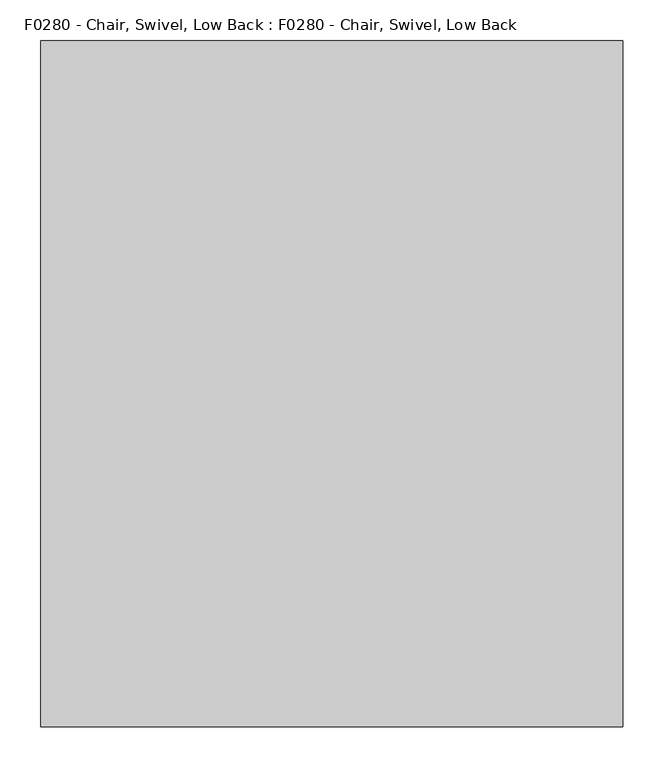
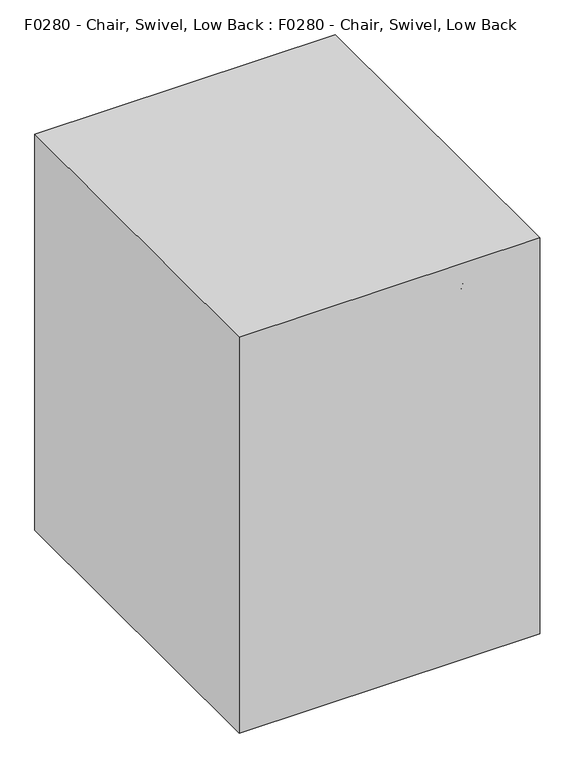
"""IFC4 building model written with IfcOpenShell, lengths in millimetres: proxy geometry, F0280 - Chair, Swivel, Low Back : F0280 - Chair, Swivel, Low Back."""

import ifcopenshell
import ifcopenshell.guid

model = None  # the IFC model being written
_history = None  # IfcOwnerHistory: only IFC2X3 demands one
_inside = {}  # id of a spatial element -> (the spatial element, [elements in it])
_under = {}  # id of a project, library or spatial element -> (it, [spatial elements below it])
_declared = {}  # id of a project -> (the project, [libraries it declares])
_typed = {}  # id of a type object -> (the type object, [elements of that type])
_made_of = {}  # id of a material, layer set ... -> (it, [elements and type objects made of it])


def new_model(schema):
    """Start an empty IFC model of exactly this schema.

    Asked for "IFC4X3", IfcOpenShell would pick the latest addendum, in which some entities
    have other attributes; the version numbers below select the first issue.
    IFC2X3 requires an IfcOwnerHistory on every rooted entity: one is made here for all.
    """
    global model, _history
    if schema == "IFC4X3":
        model = ifcopenshell.file(schema_version=(4, 3, 0, 0))
    else:
        model = ifcopenshell.file(schema=schema)
    _inside.clear()
    _under.clear()
    _declared.clear()
    _typed.clear()
    _made_of.clear()
    _history = None
    if model.schema == "IFC2X3":
        org = make("IfcOrganization", Name="unknown")
        user = make(
            "IfcPersonAndOrganization",
            ThePerson=make("IfcPerson", FamilyName="unknown"),
            TheOrganization=org,
        )
        app = make(
            "IfcApplication",
            ApplicationDeveloper=org,
            Version="unknown",
            ApplicationFullName="unknown",
            ApplicationIdentifier="unknown",
        )
        _history = make(
            "IfcOwnerHistory",
            OwningUser=user,
            OwningApplication=app,
            ChangeAction="ADDED",
            CreationDate=0,
        )
    return model


def make(cls, **values):
    """One entity of the class cls with the attributes given. An attribute that is None is left unset."""
    return model.create_entity(
        cls, **{name: value for name, value in values.items() if value is not None}
    )


def rooted(cls, **values):
    """An entity with a GlobalId (a new one), such as an element, a storey or a relation."""
    return make(cls, GlobalId=ifcopenshell.guid.new(), OwnerHistory=_history, **values)


def si_unit(unit_type, name, prefix=None):
    """IfcSIUnit, for example si_unit("LENGTHUNIT", "METRE", prefix="MILLI")."""
    return make("IfcSIUnit", UnitType=unit_type, Prefix=prefix, Name=name)


def assignment(units):
    """IfcUnitAssignment: the units of a project."""
    return None if units is None else make("IfcUnitAssignment", Units=units)


def point(xyz):
    """IfcCartesianPoint."""
    return None if xyz is None else make("IfcCartesianPoint", Coordinates=xyz)


def direction(xyz):
    """IfcDirection."""
    return None if xyz is None else make("IfcDirection", DirectionRatios=xyz)


def frame(location, z_axis=None, x_axis=None):
    """IfcAxis2Placement3D, a coordinate frame: its origin and axes. An axis left out is left unset."""
    return make(
        "IfcAxis2Placement3D",
        Location=point(location),
        Axis=direction(z_axis),
        RefDirection=direction(x_axis),
    )


def frame_2d(location, x_axis=None):
    """IfcAxis2Placement2D, a coordinate frame in the plane: its origin and x axis."""
    return make(
        "IfcAxis2Placement2D", Location=point(location), RefDirection=direction(x_axis)
    )


def origin():
    """The frame at (0, 0, 0) with its axes left unset."""
    return frame((0.0, 0.0, 0.0))


def origin_with_axes():
    """The frame at (0, 0, 0) with the z axis (0, 0, 1) and the x axis (1, 0, 0) written out."""
    return frame((0.0, 0.0, 0.0), z_axis=(0.0, 0.0, 1.0), x_axis=(1.0, 0.0, 0.0))


def origin_2d():
    """The frame at (0, 0) in the plane with its x axis left unset."""
    return frame_2d((0.0, 0.0))


def place(relative_to, where):
    """IfcLocalPlacement: puts the frame where relative to a parent placement (None: the world)."""
    return make(
        "IfcLocalPlacement", PlacementRelTo=relative_to, RelativePlacement=where
    )


def context(
    kind, dimensions, precision=None, world=None, true_north=None, identifier=None
):
    """IfcGeometricRepresentationContext, for example the 3D "Model" context."""
    return make(
        "IfcGeometricRepresentationContext",
        ContextIdentifier=identifier,
        ContextType=kind,
        CoordinateSpaceDimension=dimensions,
        Precision=precision,
        WorldCoordinateSystem=world,
        TrueNorth=true_north,
    )


def project(units=None, contexts=None):
    """IfcProject with its units and contexts."""
    return rooted(
        "IfcProject",
        Name="project",
        RepresentationContexts=contexts,
        UnitsInContext=assignment(units),
    )


def spatial(cls, under=None, at=None, **own):
    """A site, building, storey or space (cls), placed at a placement, below another one or the project."""
    s = rooted(cls, ObjectPlacement=at, **own)
    if under is not None:
        _under.setdefault(under.id(), (under, []))[1].append(s)
    return s


def polyline(points):
    """IfcPolyline through the points."""
    return make("IfcPolyline", Points=[point(p) for p in points])


def circle_curve(where, radius):
    """IfcCircle in the frame where."""
    return make("IfcCircle", Position=where, Radius=radius)


def ellipse_curve(where, semi_axis1, semi_axis2):
    """IfcEllipse in the frame where."""
    return make(
        "IfcEllipse", Position=where, SemiAxis1=semi_axis1, SemiAxis2=semi_axis2
    )


def trimmed(basis, trim1, trim2, sense, master):
    """IfcTrimmedCurve: the piece of a basis curve between two trims."""
    return make(
        "IfcTrimmedCurve",
        BasisCurve=basis,
        Trim1=trim1,
        Trim2=trim2,
        SenseAgreement=sense,
        MasterRepresentation=master,
    )


def segment(curve, same_sense, transition):
    """IfcCompositeCurveSegment."""
    return make(
        "IfcCompositeCurveSegment",
        Transition=transition,
        SameSense=same_sense,
        ParentCurve=curve,
    )


def composite_curve(segments, self_intersect=None):
    """IfcCompositeCurve: segments joined end to end."""
    return make("IfcCompositeCurve", Segments=segments, SelfIntersect=self_intersect)


def outline(outer, holes=None, kind="AREA"):
    """IfcArbitraryClosedProfileDef: a profile drawn as a closed curve; with holes, ...WithVoids."""
    if holes is None:
        return make("IfcArbitraryClosedProfileDef", ProfileType=kind, OuterCurve=outer)
    return make(
        "IfcArbitraryProfileDefWithVoids",
        ProfileType=kind,
        OuterCurve=outer,
        InnerCurves=holes,
    )


def extrude(swept, where, along, depth):
    """IfcExtrudedAreaSolid: the profile swept, set in the frame where, extruded along a direction by depth."""
    return make(
        "IfcExtrudedAreaSolid",
        SweptArea=swept,
        Position=where,
        ExtrudedDirection=direction(along),
        Depth=depth,
    )


def shape(context_of_items, identifier, shape_type, items):
    """IfcShapeRepresentation: the items that make up one representation, for example the "Body"."""
    return make(
        "IfcShapeRepresentation",
        ContextOfItems=context_of_items,
        RepresentationIdentifier=identifier,
        RepresentationType=shape_type,
        Items=items,
    )


def source(mapping_origin, context_of_items, identifier, shape_type, items):
    """IfcRepresentationMap: a shape defined once, which mapped items show again and again."""
    return make(
        "IfcRepresentationMap",
        MappingOrigin=mapping_origin,
        MappedRepresentation=shape(context_of_items, identifier, shape_type, items),
    )


def transform(
    local_origin,
    x_axis=None,
    y_axis=None,
    z_axis=None,
    scale=None,
    scale2=None,
    scale3=None,
    uniform=True,
):
    """IfcCartesianTransformationOperator3D, or its non-uniform kind. x_axis, y_axis, z_axis: its Axis1, 2, 3."""
    if uniform:
        return make(
            "IfcCartesianTransformationOperator3D",
            Axis1=direction(x_axis),
            Axis2=direction(y_axis),
            LocalOrigin=point(local_origin),
            Scale=scale,
            Axis3=direction(z_axis),
        )
    return make(
        "IfcCartesianTransformationOperator3DnonUniform",
        Axis1=direction(x_axis),
        Axis2=direction(y_axis),
        LocalOrigin=point(local_origin),
        Scale=scale,
        Axis3=direction(z_axis),
        Scale2=scale2,
        Scale3=scale3,
    )


def mapped(mapping_source, mapping_target):
    """IfcMappedItem: shows the shape of a source again, moved by a transform."""
    return make(
        "IfcMappedItem", MappingSource=mapping_source, MappingTarget=mapping_target
    )


def made_of(thing, what):
    """Note that an element or type object is made of a material, layer set ...; save() writes the relation."""
    if what is not None:
        _made_of.setdefault(what.id(), (what, []))[1].append(thing)
    return thing


def element(
    cls,
    number,
    at=None,
    inside=None,
    cuts=None,
    type_object=None,
    material=None,
    context=None,
    identifier="Body",
    shape_type=None,
    held_by="IfcProductDefinitionShape",
    body=None,
    shapes=None,
    **own,
):
    """One element of the class cls, such as IfcWall. Its Tag is "e" and its number.

    at: its placement. inside: the storey or other place that contains it. cuts: it is an
    opening in that element (IfcRelVoidsElement). A single representation is given by context,
    identifier, shape_type and body (its items); several are given by shapes. held_by: the class
    of the entity that holds the representations. save() writes the other relations.
    """
    e = rooted(cls, Tag="e%d" % number, ObjectPlacement=at, **own)
    if body is not None:
        shapes = [shape(context, identifier, shape_type, body)]
    if shapes is not None:
        e.Representation = make(held_by, Representations=shapes)
    if inside is not None:
        _inside.setdefault(inside.id(), (inside, []))[1].append(e)
    if cuts is not None:
        rooted(
            "IfcRelVoidsElement", RelatingBuildingElement=cuts, RelatedOpeningElement=e
        )
    if type_object is not None:
        _typed.setdefault(type_object.id(), (type_object, []))[1].append(e)
    return made_of(e, material)


def aggregate(whole, parts):
    """IfcRelAggregates: a whole, such as a stair, and the parts it consists of."""
    return rooted("IfcRelAggregates", RelatingObject=whole, RelatedObjects=parts)


def save(model, path):
    """Write the relations noted so far, then the file.

    IfcRelAggregates (storeys below a building ...), IfcRelContainedInSpatialStructure (elements
    in a storey), IfcRelDefinesByType, IfcRelAssociatesMaterial and IfcRelDeclares: one each for
    every whole, place, type object, material and project.
    """
    for whole, parts in _under.values():
        aggregate(whole, parts)
    for where, things in _inside.values():
        rooted(
            "IfcRelContainedInSpatialStructure",
            RelatedElements=things,
            RelatingStructure=where,
        )
    for kind, things in _typed.values():
        rooted("IfcRelDefinesByType", RelatedObjects=things, RelatingType=kind)
    for what, things in _made_of.values():
        rooted("IfcRelAssociatesMaterial", RelatedObjects=things, RelatingMaterial=what)
    for by, libraries in _declared.values():
        rooted("IfcRelDeclares", RelatingContext=by, RelatedDefinitions=libraries)
    model.write(path)


def plane_surface(at):
    """IfcPlane: the flat surface through the origin of the frame at, square to its z axis."""
    return make("IfcPlane", Position=at)


def cylinder_surface(at, radius):
    """IfcCylindricalSurface: all points at the distance radius from the z axis of the frame at."""
    return make("IfcCylindricalSurface", Position=at, Radius=radius)


def revolved_surface(curve, axis_point, axis_direction):
    """IfcSurfaceOfRevolution: the curve turned about the line through axis_point along axis_direction."""
    return make(
        "IfcSurfaceOfRevolution",
        SweptCurve=make("IfcArbitraryOpenProfileDef", ProfileType="CURVE", Curve=curve),
        AxisPosition=make("IfcAxis1Placement", Location=point(axis_point), Axis=direction(axis_direction)),
    )


def advanced_brep(points, edges, surfaces, faces):
    """IfcAdvancedBrep: a solid bounded by faces that lie on surfaces and meet in shared edges.

    An edge is (start, end): straight between two places in points (the first is 0);
    or (start, end, curve); or (start, end, curve, False) where it runs against its curve.
    A face is (place in surfaces, loops), or (place, loops, False) where it looks against
    its surface's normal. A loop lists edges by number (the first is 1), with a minus sign
    where the edge is run from its end to its start. The first loop is the outer one.
    """
    corners = [point(p) for p in points]
    vertices = [make("IfcVertexPoint", VertexGeometry=c) for c in corners]
    made = []
    for start, end, *more in edges:
        made.append(
            make(
                "IfcEdgeCurve",
                EdgeStart=vertices[start],
                EdgeEnd=vertices[end],
                EdgeGeometry=more[0] if more else make("IfcPolyline", Points=[corners[start], corners[end]]),
                SameSense=more[1] if len(more) > 1 else True,
            )
        )
    hull = []
    for where, loops, *sense in faces:
        bounds = []
        for j, loop in enumerate(loops):
            ring = [make("IfcOrientedEdge", EdgeElement=made[abs(k) - 1], Orientation=k > 0) for k in loop]
            bounds.append(
                make(
                    "IfcFaceOuterBound" if j == 0 else "IfcFaceBound",
                    Bound=make("IfcEdgeLoop", EdgeList=ring),
                    Orientation=True,
                )
            )
        hull.append(make("IfcAdvancedFace", Bounds=bounds, FaceSurface=surfaces[where], SameSense=sense[0] if sense else True))
    return make("IfcAdvancedBrep", Outer=make("IfcClosedShell", CfsFaces=hull))


def f0280_chair_swivel_low_back_f0280_chair_swivel_low_back_8651f157(model_context):
    return source(origin(), model_context, "Body", "SolidModel", [
        advanced_brep(
        [(20.5891067, 0.9088165, 158.3164474), (12.606954, -16.2089653, 158.3164474), (12.606954, -16.2089653, 212.7487443), (20.5891067, 0.9088165, 212.7487443), (283.7284885, -121.7950923, 86.0096871), (283.7284885, -121.7950923, 57.6571213), (275.3053581, -138.7072429, 86.2220806), (287.501904, -133.9556376, 82.2734822), (275.3053581, -138.7072429, 57.8258095), (287.501904, -133.9556376, 54.689734)],
        [
            (0, 1),
            (1, 2),
            (2, 3),
            (3, 0),
            (3, 4),
            (4, 5),
            (5, 0),
            (2, 6),
            (6, 7, ellipse_curve(frame((278.918781, -129.9532617, 86.4074773), z_axis=(0.3625792018206629, -0.16907345849670724, 0.9164881276039822), x_axis=(0.8306203267741233, -0.3873246193939933, -0.40006188516396646)), 10.333389, 9.4704283)),
            (7, 4, ellipse_curve(frame((278.918781, -129.9532617, 86.4074773), z_axis=(0.3625792018206629, -0.16907345849670724, 0.9164881276039822), x_axis=(0.8306203267741233, -0.3873246193939933, -0.40006188516396646)), 10.333389, 9.4704283)),
            (1, 8),
            (8, 6),
            (5, 9, ellipse_curve(frame((278.918781, -129.9532617, 57.9730562), z_axis=(-0.2968743688836678, 0.13843479172039067, -0.9448287768380342), x_axis=(0.8563056778646188, -0.3993018953098915, -0.3275646233321667)), 10.0234334, 9.4704283)),
            (9, 8, ellipse_curve(frame((278.918781, -129.9532617, 57.9730562), z_axis=(-0.2968743688836678, 0.13843479172039067, -0.9448287768380342), x_axis=(0.8563056778646188, -0.3993018953098915, -0.3275646233321667)), 10.0234334, 9.4704283)),
            (9, 7),
        ],
        [
            plane_surface(frame((16.5980304, -7.6500744, 185.5325958), z_axis=(-0.9063077870366449, 0.42261826174071043, 0.0), x_axis=(-0.42261826174071043, -0.9063077870366449, 0.0))),
            plane_surface(frame((20.5891067, 0.9088165, 185.5325958), z_axis=(0.4226182617407104, 0.9063077870366448, 0.0), x_axis=(0.0, 0.0, 1.0))),
            plane_surface(frame((16.5980304, -7.6500744, 212.7487443), z_axis=(0.36257920182066294, -0.16907345849670727, 0.9164881276039825), x_axis=(-0.42261826174071043, -0.9063077870366449, 0.0))),
            plane_surface(frame((12.606954, -16.2089653, 185.5325958), z_axis=(-0.4226182617407102, -0.906307787036645, 0.0), x_axis=(0.0, 0.0, -1.0))),
            plane_surface(frame((16.5980304, -7.6500744, 158.3164474), z_axis=(-0.29687436888366786, 0.1384347917203907, -0.9448287768380345), x_axis=(0.42261826174071043, 0.9063077870366449, 0.0))),
            cylinder_surface(frame((278.918781, -129.9532617, 0.0), z_axis=(0.0, 0.0, -1.0000000000000002), x_axis=(-0.9063077870366449, 0.42261826174071043, 0.0)), 9.4704283),
        ],
        [
            (0, [[1, 2, 3, 4]]),
            (1, [[-4, 5, 6, 7]]),
            (2, [[-3, 8, 9, 10, -5]]),
            (3, [[-2, 11, 12, -8]]),
            (4, [[-1, -7, 13, 14, -11]]),
            (5, [[15, -9, -12, -14]]),
            (5, [[-15, -13, -6, -10]]),
        ],
    ),
        extrude(outline(composite_curve([segment(trimmed(circle_curve(frame_2d((-0.4565328, 0.2009494)), 25.4), [point((24.9434672, 0.2009494))], [point((-25.8565328, 0.2009494))], False, "CARTESIAN"), True, "CONTINUOUS"), segment(trimmed(circle_curve(frame_2d((-0.4565328, 0.2009494)), 25.4), [point((-25.8565328, 0.2009494))], [point((24.9434672, 0.2009494))], False, "CARTESIAN"), True, "CONTINUOUS")], self_intersect=False)), frame((0.0, 0.0, 154.0271692), z_axis=(0.0, 0.0, 1.0), x_axis=(1.0, 0.0, 0.0)), (0.0, 0.0, 1.0), 58.7215752),
        advanced_brep(
        [(-229.5082147, -191.2947504, 328.6387079), (232.0214447, -190.8605661, 328.5937403), (236.3508412, -215.7557493, 331.1720849), (-229.5082147, -216.926585, 331.293346), (-229.5082147, -284.2177228, 855.6310718), (-229.5082147, -307.3958289, 844.3699241), (236.3508412, -306.337077, 844.8843217), (232.0214447, -283.8251028, 855.8218273)],
        [
            (0, 1, circle_curve(frame((0.0, 1130.5045098, 191.7425871), z_axis=(0.0, 0.10301698777210262, 0.9946795967699159), x_axis=(-1.0, 0.0, 0.0)), 1348.5428628)),
            (1, 2, circle_curve(frame((232.0214447, -203.6806144, 329.9214872), z_axis=(0.0, -0.10301698777210262, -0.9946795967699159), x_axis=(-1.0, 0.0, 0.0)), 12.888621)),
            (2, 3, circle_curve(frame((0.0, 1130.5045098, 191.7425871), z_axis=(0.0, -0.10301698777210262, -0.9946795967699159), x_axis=(-1.0, 0.0, 0.0)), 1373.9428628)),
            (3, 0, circle_curve(frame((-229.5082147, -204.1106677, 329.9660269), z_axis=(0.0, -0.10301698777210262, -0.9946795967699159), x_axis=(-1.0, 0.0, 0.0)), 12.8844679)),
            (4, 5, circle_curve(frame((-229.5082147, -295.8067759, 850.0004979), z_axis=(0.0, -0.4370047614753844, 0.8994591922082082), x_axis=(-1.0, 0.0, 0.0)), 12.8844679)),
            (5, 6, circle_curve(frame((0.0, 911.0460573, 1436.3533187), z_axis=(0.0, -0.4370047614753844, 0.8994591922082082), x_axis=(-1.0, 0.0, 0.0)), 1373.9428628)),
            (6, 7, circle_curve(frame((232.0214447, -295.4178914, 850.1894385), z_axis=(0.0, -0.4370047614753844, 0.8994591922082082), x_axis=(-1.0, 0.0, 0.0)), 12.888621)),
            (7, 4, circle_curve(frame((0.0, 911.0460573, 1436.3533187), z_axis=(0.0, 0.4370047614753844, -0.8994591922082082), x_axis=(-1.0, 0.0, 0.0)), 1348.5428628)),
            (7, 1, circle_curve(frame((232.0214447, -1161.9751957, 429.1701512), z_axis=(-1.0, 0.0, 0.0), x_axis=(0.0, 0.9946795967699159, -0.10301698777210261)), 976.308987)),
            (0, 4, circle_curve(frame((-229.5082147, -1161.9751957, 429.1701512), z_axis=(1.0, 0.0, 0.0), x_axis=(0.0, 0.9946795967699159, -0.10301698777210261)), 975.8724803)),
            (6, 2, circle_curve(frame((236.3508412, -1161.9751957, 429.1701512), z_axis=(-1.0, 0.0, 0.0), x_axis=(0.0, 0.9946795967699159, -0.10301698777210261)), 951.280643)),
            (5, 3, circle_curve(frame((-229.5082147, -1161.9751957, 429.1701512), z_axis=(-1.0, 0.0, 0.0), x_axis=(0.0, 0.9946795967699159, -0.10301698777210261)), 950.1035446)),
        ],
        [
            plane_surface(frame((-317.5, -173.1564347, 326.7601586), z_axis=(0.0, -0.10301698777210258, -0.994679596769916), x_axis=(-1.0, 0.0, 0.0))),
            plane_surface(frame((-317.5, -267.815783, 863.6), z_axis=(0.0, -0.4370047614753844, 0.8994591922082082), x_axis=(-1.0, 0.0, 0.0))),
            revolved_surface(trimmed(ellipse_curve(frame((0.0, 1130.5045098, 191.7425871), z_axis=(0.0, 0.10301698777210262, 0.9946795967699159), x_axis=(-1.0, 0.0, 0.0)), 1348.5428628, 1348.5428628), [point((-229.5082147, -191.2947504, 328.6387079))], [point((232.0214447, -190.8605661, 328.5937403))], True, "CARTESIAN"), (-317.5, -1161.9751957, 429.1701512), (1.0, 0.0, 0.0)),
            revolved_surface(trimmed(ellipse_curve(frame((232.0214447, -203.6806144, 329.9214872), z_axis=(0.0, -0.10301698777210262, -0.9946795967699159), x_axis=(-1.0, 0.0, 0.0)), 12.888621, 12.888621), [point((232.0214447, -190.8605661, 328.5937403))], [point((236.3508412, -215.7557493, 331.1720849))], True, "CARTESIAN"), (-317.5, -1161.9751957, 429.1701512), (1.0, 0.0, 0.0)),
            revolved_surface(trimmed(ellipse_curve(frame((0.0, 1130.5045098, 191.7425871), z_axis=(0.0, -0.10301698777210262, -0.9946795967699159), x_axis=(-1.0, 0.0, 0.0)), 1373.9428628, 1373.9428628), [point((236.3508412, -215.7557493, 331.1720849))], [point((-229.5082147, -216.926585, 331.293346))], True, "CARTESIAN"), (-317.5, -1161.9751957, 429.1701512), (1.0, 0.0, 0.0)),
            revolved_surface(trimmed(ellipse_curve(frame((-229.5082147, -204.1106677, 329.9660269), z_axis=(0.0, -0.10301698777210262, -0.9946795967699159), x_axis=(-1.0, 0.0, 0.0)), 12.8844679, 12.8844679), [point((-229.5082147, -216.926585, 331.293346))], [point((-229.5082147, -191.2947504, 328.6387079))], True, "CARTESIAN"), (-317.5, -1161.9751957, 429.1701512), (1.0, 0.0, 0.0)),
        ],
        [
            (0, [[1, 2, 3, 4]]),
            (1, [[5, 6, 7, 8]]),
            (2, [[9, -1, 10, -8]]),
            (3, [[11, -2, -9, -7]]),
            (4, [[12, -3, -11, -6]]),
            (5, [[-10, -4, -12, -5]]),
        ],
    ),
        extrude(outline(composite_curve([segment(polyline([(-213.079753, -174.0379297), (-213.079753, 182.9075832)]), True, "CONTINUOUS"), segment(trimmed(circle_curve(frame_2d((-186.3342402, 182.9075832)), 26.7455128), [point((-213.079753, 182.9075832))], [point((-186.3342402, 209.653096))], False, "CARTESIAN"), True, "CONTINUOUS"), segment(polyline([(-186.3342402, 209.653096), (194.6657598, 209.653096)]), True, "CONTINUOUS"), segment(trimmed(circle_curve(frame_2d((194.6657598, 182.9075832)), 26.7455128), [point((194.6657598, 209.653096))], [point((221.4112726, 182.9075832))], False, "CARTESIAN"), True, "CONTINUOUS"), segment(polyline([(221.4112726, 182.9075832), (221.4112726, -174.0379297), (-213.079753, -174.0379297)]), True, "CONTINUOUS")], self_intersect=False)), frame((0.0, 0.0, 324.0440254), z_axis=(0.0, 0.0, 1.0), x_axis=(1.0, 0.0, 0.0)), (0.0, 0.0, 1.0), 67.8491407),
        advanced_brep(
        [(-213.079753, -172.6924168, 391.8931661), (-211.7342402, -174.0379297, 391.8931661), (-211.7342402, -174.0379297, 324.0440254), (-213.079753, -172.6924168, 324.0440254), (-213.079753, 182.9075832, 324.0440254), (-213.079753, 182.9075832, 391.8931661), (-186.3342402, 209.653096, 391.8931661), (-186.3342402, 209.653096, 324.0440254), (194.6657598, 209.653096, 324.0440254), (194.6657598, 209.653096, 391.8931661), (221.4112726, 182.9075832, 391.8931661), (221.4112726, 182.9075832, 324.0440254), (221.4112726, -172.6924168, 324.0440254), (221.4112726, -172.6924168, 391.8931661), (220.0657598, -174.0379297, 391.8931661), (220.0657598, -174.0379297, 324.0440254)],
        [
            (0, 1, circle_curve(frame((-211.7342402, -172.6924168, 391.8931661), z_axis=(0.0, 0.0, 1.0), x_axis=(0.0, -1.0, 0.0)), 1.3455128)),
            (1, 2),
            (2, 3, circle_curve(frame((-211.7342402, -172.6924168, 324.0440254), z_axis=(0.0, 0.0, -1.0), x_axis=(0.0, -1.0, 0.0)), 1.3455128)),
            (3, 0),
            (2, 1, circle_curve(frame((-211.7342402, -174.0379297, 357.9685958), z_axis=(-1.0, 0.0, 0.0), x_axis=(0.0, 1.0, 0.0)), 33.9245703)),
            (0, 3, circle_curve(frame((-213.079753, -172.6924168, 357.9685958), z_axis=(0.0, -1.0, 0.0), x_axis=(1.0, 0.0, 0.0)), 33.9245703)),
            (3, 4),
            (4, 5),
            (5, 0),
            (5, 4, circle_curve(frame((-213.079753, 182.9075832, 357.9685958), z_axis=(0.0, -1.0, 0.0), x_axis=(1.0, 0.0, 0.0)), 33.9245703)),
            (6, 5, circle_curve(frame((-186.3342402, 182.9075832, 391.8931661), z_axis=(0.0, 0.0, 1.0), x_axis=(-1.0, 0.0, 0.0)), 26.7455128)),
            (4, 7, circle_curve(frame((-186.3342402, 182.9075832, 324.0440254), z_axis=(0.0, 0.0, -1.0), x_axis=(-1.0, 0.0, 0.0)), 26.7455128)),
            (7, 6),
            (6, 7, circle_curve(frame((-186.3342402, 209.653096, 357.9685958), z_axis=(-1.0, 0.0, 0.0), x_axis=(0.0, -1.0, 0.0)), 33.9245703)),
            (7, 8),
            (8, 9),
            (9, 6),
            (9, 8, circle_curve(frame((194.6657598, 209.653096, 357.9685958), z_axis=(-1.0, 0.0, 0.0), x_axis=(0.0, -1.0, 0.0)), 33.9245703)),
            (10, 9, circle_curve(frame((194.6657598, 182.9075832, 391.8931661), z_axis=(0.0, 0.0, 1.0), x_axis=(0.0, 1.0, 0.0)), 26.7455128)),
            (8, 11, circle_curve(frame((194.6657598, 182.9075832, 324.0440254), z_axis=(0.0, 0.0, -1.0), x_axis=(0.0, 1.0, 0.0)), 26.7455128)),
            (11, 10),
            (10, 11, circle_curve(frame((221.4112726, 182.9075832, 357.9685958), z_axis=(0.0, 1.0, 0.0), x_axis=(-1.0, 0.0, 0.0)), 33.9245703)),
            (11, 12),
            (12, 13),
            (13, 10),
            (13, 12, circle_curve(frame((221.4112726, -172.6924168, 357.9685958), z_axis=(0.0, 1.0, 0.0), x_axis=(-1.0, 0.0, 0.0)), 33.9245703)),
            (14, 13, circle_curve(frame((220.0657598, -172.6924168, 391.8931661), z_axis=(0.0, 0.0, 1.0), x_axis=(1.0, 0.0, 0.0)), 1.3455128)),
            (12, 15, circle_curve(frame((220.0657598, -172.6924168, 324.0440254), z_axis=(0.0, 0.0, -1.0), x_axis=(1.0, 0.0, 0.0)), 1.3455128)),
            (15, 14),
            (14, 15, circle_curve(frame((220.0657598, -174.0379297, 357.9685958), z_axis=(1.0, 0.0, 0.0), x_axis=(0.0, 1.0, 0.0)), 33.9245703)),
            (15, 2),
            (1, 14),
        ],
        [
            revolved_surface(polyline([(-211.7342402, -174.03792959999998, 324.0440254), (-211.7342402, -174.03792959999998, 391.8931661)]), (-211.7342402, -172.6924168, 0.0), (0.0, 0.0, -1.0)),
            revolved_surface(trimmed(ellipse_curve(frame((-211.7342402, -174.0379297, 357.9685958), z_axis=(1.0, 0.0, 0.0), x_axis=(0.0, 1.0, 0.0)), 33.9245703, 33.9245703), [point((-211.7342402, -174.0379297, 391.8931661))], [point((-211.7342402, -174.0379297, 324.0440254))], True, "CARTESIAN"), (-211.7342402, -172.6924168, 0.0), (0.0, 0.0, -1.0)),
            plane_surface(frame((-213.079753, -172.6924168, 324.0440254), z_axis=(1.0, 0.0, 0.0), x_axis=(0.0, 1.0, 0.0))),
            cylinder_surface(frame((-213.079753, -172.6924168, 357.9685958), z_axis=(0.0, -1.0, 0.0), x_axis=(1.0, 0.0, 0.0)), 33.9245703),
            revolved_surface(polyline([(-213.079753, 182.9075832, 324.0440254), (-213.079753, 182.9075832, 391.8931661)]), (-186.3342402, 182.9075832, 0.0), (0.0, 0.0, -1.0)),
            revolved_surface(trimmed(ellipse_curve(frame((-213.079753, 182.9075832, 357.9685958), z_axis=(0.0, -1.0, 0.0), x_axis=(1.0, 0.0, 0.0)), 33.9245703, 33.9245703), [point((-213.079753, 182.9075832, 391.8931661))], [point((-213.079753, 182.9075832, 324.0440254))], True, "CARTESIAN"), (-186.3342402, 182.9075832, 0.0), (0.0, 0.0, -1.0)),
            plane_surface(frame((-186.3342402, 209.653096, 324.0440254), z_axis=(0.0, -1.0, 0.0), x_axis=(1.0, 0.0, 0.0))),
            cylinder_surface(frame((-186.3342402, 209.653096, 357.9685958), z_axis=(-1.0, 0.0, 0.0), x_axis=(0.0, -1.0, 0.0)), 33.9245703),
            revolved_surface(polyline([(194.6657598, 209.653096, 324.0440254), (194.6657598, 209.653096, 391.8931661)]), (194.6657598, 182.9075832, 0.0), (0.0, 0.0, -1.0)),
            revolved_surface(trimmed(ellipse_curve(frame((194.6657598, 209.653096, 357.9685958), z_axis=(-1.0, 0.0, 0.0), x_axis=(0.0, -1.0, 0.0)), 33.9245703, 33.9245703), [point((194.6657598, 209.653096, 391.8931661))], [point((194.6657598, 209.653096, 324.0440254))], True, "CARTESIAN"), (194.6657598, 182.9075832, 0.0), (0.0, 0.0, -1.0)),
            plane_surface(frame((221.4112726, 182.9075832, 324.0440254), z_axis=(-1.0, 0.0, 0.0), x_axis=(0.0, -1.0, 0.0))),
            cylinder_surface(frame((221.4112726, 182.9075832, 357.9685958), z_axis=(0.0, 1.0, 0.0), x_axis=(-1.0, 0.0, 0.0)), 33.9245703),
            revolved_surface(polyline([(221.4112726, -172.6924168, 324.0440254), (221.4112726, -172.6924168, 391.8931661)]), (220.0657598, -172.6924168, 0.0), (0.0, 0.0, -1.0)),
            revolved_surface(trimmed(ellipse_curve(frame((221.4112726, -172.6924168, 357.9685958), z_axis=(0.0, 1.0, 0.0), x_axis=(-1.0, 0.0, 0.0)), 33.9245703, 33.9245703), [point((221.4112726, -172.6924168, 391.8931661))], [point((221.4112726, -172.6924168, 324.0440254))], True, "CARTESIAN"), (220.0657598, -172.6924168, 0.0), (0.0, 0.0, -1.0)),
            plane_surface(frame((220.0657598, -174.0379297, 324.0440254), z_axis=(0.0, 1.0, 0.0), x_axis=(-1.0, 0.0, 0.0))),
            cylinder_surface(frame((220.0657598, -174.0379297, 357.9685958), z_axis=(1.0, 0.0, 0.0), x_axis=(0.0, 1.0, 0.0)), 33.9245703),
        ],
        [
            (0, [[1, 2, 3, 4]]),
            (1, [[-3, 5, -1, 6]]),
            (2, [[-4, 7, 8, 9]]),
            (3, [[-6, -9, 10, -7]]),
            (4, [[11, -8, 12, 13]]),
            (5, [[-12, -10, -11, 14]]),
            (6, [[-13, 15, 16, 17]]),
            (7, [[-14, -17, 18, -15]]),
            (8, [[19, -16, 20, 21]]),
            (9, [[-20, -18, -19, 22]]),
            (10, [[-21, 23, 24, 25]]),
            (11, [[-22, -25, 26, -23]]),
            (12, [[27, -24, 28, 29]]),
            (13, [[-28, -26, -27, 30]]),
            (14, [[-29, 31, -2, 32]]),
            (15, [[-30, -32, -5, -31]]),
        ],
    ),
        extrude(outline(composite_curve([segment(trimmed(circle_curve(origin_2d(), 12.7), [point((12.7, 0.0))], [point((-12.7, 0.0))], False, "CARTESIAN"), True, "CONTINUOUS"), segment(trimmed(circle_curve(origin_2d(), 12.7), [point((-12.7, 0.0))], [point((12.7, 0.0))], False, "CARTESIAN"), True, "CONTINUOUS")], self_intersect=False)), frame((0.0, 0.0, 212.7487443), z_axis=(0.0, 0.0, 1.0), x_axis=(1.0, 0.0, 0.0)), (0.0, 0.0, 1.0), 66.217703),
        extrude(outline(polyline([(355.6, 419.1), (355.6, -419.1), (-355.6, -419.1), (-355.6, 419.1), (355.6, 419.1)])), origin_with_axes(), (0.0, 0.0, 1.0), 990.6),
    ])


if __name__ == "__main__":
    model = new_model("IFC4")
    model_context = context("Model", 3, world=origin())
    ifc_project = project(units=[si_unit("LENGTHUNIT", "METRE", prefix="MILLI")], contexts=[model_context])
    site = spatial("IfcSite", under=ifc_project)
    building = spatial("IfcBuilding", under=site)
    placement = place(None, origin())
    f0280_chair_swivel_low_back_f0280_chair_swivel_low_back_shape = f0280_chair_swivel_low_back_f0280_chair_swivel_low_back_8651f157(model_context)
    element("IfcBuildingElementProxy", 1, Name="F0280 - Chair, Swivel, Low Back : F0280 - Chair, Swivel, Low Back", ObjectType="F0280 - Chair, Swivel, Low Back : F0280 - Chair, Swivel, Low Back", at=placement, inside=building, context=model_context, shape_type="MappedRepresentation", body=[
        mapped(f0280_chair_swivel_low_back_f0280_chair_swivel_low_back_shape, transform((0.0, 0.0, 0.0), x_axis=(1.0, 0.0, 0.0), y_axis=(0.0, 1.0, 0.0), z_axis=(0.0, 0.0, 1.0))),
    ])
    save(model, "model.ifc")

# Revit data of these elements
# Type "F0280 - Chair, Swivel, Low Back : F0280 - Chair, Swivel, Low Back"
#   Watts2 = "0"
#   Watts1 = "0"
#   Unit_Issue = "EA"
#   UTIL_6_Misc = "-"
#   UTIL_5_NonMedGas = "-"
#   UTIL_4_MiscGas = "-"
#   UTIL_3_MedGas = "-"
#   UTIL_2_Elec = "-"
#   UTIL_1_WaterDrain = "-"
#   Nomenclature = "Chair, Swivel, Low Back"
#   NSN = "7110"
#   Location [instance default] = ""
#   JSN = "F0280"
#   Fund_Source_VA = "-"
#   Fund_Source_Navy = "-"
#   Fund_Source_Army = "-"
#   Fund_Source_AF = "-"
#   ELEC_Volts2 = "0"
#   ELEC_Volts1 = "0"
#   ELEC_Phase2 = "0"
#   ELEC_Phase1 = "0"
#   ELEC_HertzSwitch = "0"
#   ELEC_HertzDependent = "0"
#   ELEC_Hertz = "0"
#   ELEC_Amps2 = "0"
#   ELEC_Amps1 = "0"
#   DetailDescription = "Low back contemporary swivel chair, 37\" high X 25\" wide X 31\" deep with a five (5) caster swivel base, arms and foam padded seat and back upholstered with either woven textile fabric or vinyl."
#   CAT_VA = "C"
#   CAT_Navy = "C"
#   CAT_IHS = "-"
#   CAT_Army = "C"
#   CAT_AF = "C"
#   BTUperhour = "0"
#   Weight_IP = 49
#   DIM_Width_IP = 2' - 4"
#   DIM_Height_IP = 3' - 3"
#   DIM_Depth_IP = 2' - 9"
#   Assembly Code = ""
# Element 1 (IfcBuildingElementProxy, "F0280 - Chair, Swivel, Low Back : F0280 - Chair, Swivel, Low Back")
#   Materials on its faces: "00 - bernhardt blitz - base", "00 - bernhardt blitz - Seat Fabric", "00 - bernhardt blitz - wheels", "00 - bernhardt blitz - arms", "00 - bernhardt blitz - mechanic", "00 - bernhardt blitz - Back Fabric", "EquipSpace"
# Materials
#   "00 - bernhardt blitz - base": class "Miscellaneous", colour RGB 192 192 192, transparency 0
#   "00 - bernhardt blitz - Seat Fabric": class "Miscellaneous", colour RGB 188 173 117, transparency 0
#   "00 - bernhardt blitz - wheels": class "Miscellaneous", colour RGB 51 51 51, transparency 0
#   "00 - bernhardt blitz - arms": class "Miscellaneous", colour RGB 51 51 51, transparency 0
#   "00 - bernhardt blitz - mechanic": class "Miscellaneous", colour RGB 62 62 62, transparency 0
#   "00 - bernhardt blitz - Back Fabric": class "Miscellaneous", colour RGB 93 93 93, transparency 0
#   "EquipSpace": class "Unassigned", colour RGB 221 217 195, transparency 0.5
